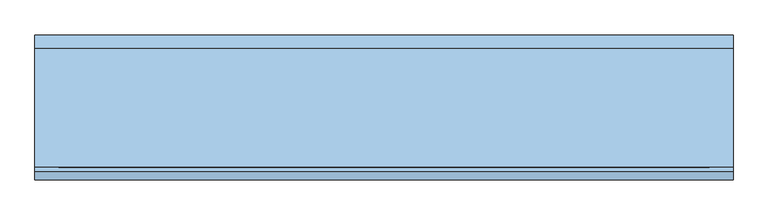
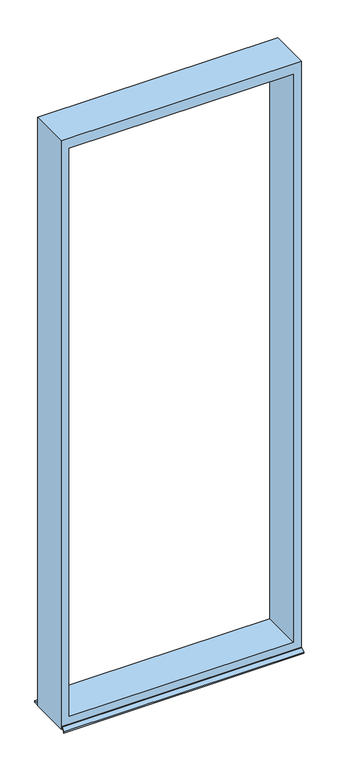
"""IFC4 building model written with IfcOpenShell, lengths in millimetres: window geometry, Fenster - Festverglasung : Feste Verglasung 4.58 x 1.77 3 2 2 2."""

import ifcopenshell
import ifcopenshell.guid

model = None  # the IFC model being written
_history = None  # IfcOwnerHistory: only IFC2X3 demands one
_inside = {}  # id of a spatial element -> (the spatial element, [elements in it])
_under = {}  # id of a project, library or spatial element -> (it, [spatial elements below it])
_declared = {}  # id of a project -> (the project, [libraries it declares])
_typed = {}  # id of a type object -> (the type object, [elements of that type])
_made_of = {}  # id of a material, layer set ... -> (it, [elements and type objects made of it])


def new_model(schema):
    """Start an empty IFC model of exactly this schema.

    Asked for "IFC4X3", IfcOpenShell would pick the latest addendum, in which some entities
    have other attributes; the version numbers below select the first issue.
    IFC2X3 requires an IfcOwnerHistory on every rooted entity: one is made here for all.
    """
    global model, _history
    if schema == "IFC4X3":
        model = ifcopenshell.file(schema_version=(4, 3, 0, 0))
    else:
        model = ifcopenshell.file(schema=schema)
    _inside.clear()
    _under.clear()
    _declared.clear()
    _typed.clear()
    _made_of.clear()
    _history = None
    if model.schema == "IFC2X3":
        org = make("IfcOrganization", Name="unknown")
        user = make(
            "IfcPersonAndOrganization",
            ThePerson=make("IfcPerson", FamilyName="unknown"),
            TheOrganization=org,
        )
        app = make(
            "IfcApplication",
            ApplicationDeveloper=org,
            Version="unknown",
            ApplicationFullName="unknown",
            ApplicationIdentifier="unknown",
        )
        _history = make(
            "IfcOwnerHistory",
            OwningUser=user,
            OwningApplication=app,
            ChangeAction="ADDED",
            CreationDate=0,
        )
    return model


def make(cls, **values):
    """One entity of the class cls with the attributes given. An attribute that is None is left unset."""
    return model.create_entity(
        cls, **{name: value for name, value in values.items() if value is not None}
    )


def rooted(cls, **values):
    """An entity with a GlobalId (a new one), such as an element, a storey or a relation."""
    return make(cls, GlobalId=ifcopenshell.guid.new(), OwnerHistory=_history, **values)


def si_unit(unit_type, name, prefix=None):
    """IfcSIUnit, for example si_unit("LENGTHUNIT", "METRE", prefix="MILLI")."""
    return make("IfcSIUnit", UnitType=unit_type, Prefix=prefix, Name=name)


def assignment(units):
    """IfcUnitAssignment: the units of a project."""
    return None if units is None else make("IfcUnitAssignment", Units=units)


def point(xyz):
    """IfcCartesianPoint."""
    return None if xyz is None else make("IfcCartesianPoint", Coordinates=xyz)


def direction(xyz):
    """IfcDirection."""
    return None if xyz is None else make("IfcDirection", DirectionRatios=xyz)


def frame(location, z_axis=None, x_axis=None):
    """IfcAxis2Placement3D, a coordinate frame: its origin and axes. An axis left out is left unset."""
    return make(
        "IfcAxis2Placement3D",
        Location=point(location),
        Axis=direction(z_axis),
        RefDirection=direction(x_axis),
    )


def origin():
    """The frame at (0, 0, 0) with its axes left unset."""
    return frame((0.0, 0.0, 0.0))


def place(relative_to, where):
    """IfcLocalPlacement: puts the frame where relative to a parent placement (None: the world)."""
    return make(
        "IfcLocalPlacement", PlacementRelTo=relative_to, RelativePlacement=where
    )


def context(
    kind, dimensions, precision=None, world=None, true_north=None, identifier=None
):
    """IfcGeometricRepresentationContext, for example the 3D "Model" context."""
    return make(
        "IfcGeometricRepresentationContext",
        ContextIdentifier=identifier,
        ContextType=kind,
        CoordinateSpaceDimension=dimensions,
        Precision=precision,
        WorldCoordinateSystem=world,
        TrueNorth=true_north,
    )


def project(units=None, contexts=None):
    """IfcProject with its units and contexts."""
    return rooted(
        "IfcProject",
        Name="project",
        RepresentationContexts=contexts,
        UnitsInContext=assignment(units),
    )


def spatial(cls, under=None, at=None, **own):
    """A site, building, storey or space (cls), placed at a placement, below another one or the project."""
    s = rooted(cls, ObjectPlacement=at, **own)
    if under is not None:
        _under.setdefault(under.id(), (under, []))[1].append(s)
    return s


def polyline(points):
    """IfcPolyline through the points."""
    return make("IfcPolyline", Points=[point(p) for p in points])


def outline(outer, holes=None, kind="AREA"):
    """IfcArbitraryClosedProfileDef: a profile drawn as a closed curve; with holes, ...WithVoids."""
    if holes is None:
        return make("IfcArbitraryClosedProfileDef", ProfileType=kind, OuterCurve=outer)
    return make(
        "IfcArbitraryProfileDefWithVoids",
        ProfileType=kind,
        OuterCurve=outer,
        InnerCurves=holes,
    )


def extrude(swept, where, along, depth):
    """IfcExtrudedAreaSolid: the profile swept, set in the frame where, extruded along a direction by depth."""
    return make(
        "IfcExtrudedAreaSolid",
        SweptArea=swept,
        Position=where,
        ExtrudedDirection=direction(along),
        Depth=depth,
    )


def shape(context_of_items, identifier, shape_type, items):
    """IfcShapeRepresentation: the items that make up one representation, for example the "Body"."""
    return make(
        "IfcShapeRepresentation",
        ContextOfItems=context_of_items,
        RepresentationIdentifier=identifier,
        RepresentationType=shape_type,
        Items=items,
    )


def source(mapping_origin, context_of_items, identifier, shape_type, items):
    """IfcRepresentationMap: a shape defined once, which mapped items show again and again."""
    return make(
        "IfcRepresentationMap",
        MappingOrigin=mapping_origin,
        MappedRepresentation=shape(context_of_items, identifier, shape_type, items),
    )


def transform(
    local_origin,
    x_axis=None,
    y_axis=None,
    z_axis=None,
    scale=None,
    scale2=None,
    scale3=None,
    uniform=True,
):
    """IfcCartesianTransformationOperator3D, or its non-uniform kind. x_axis, y_axis, z_axis: its Axis1, 2, 3."""
    if uniform:
        return make(
            "IfcCartesianTransformationOperator3D",
            Axis1=direction(x_axis),
            Axis2=direction(y_axis),
            LocalOrigin=point(local_origin),
            Scale=scale,
            Axis3=direction(z_axis),
        )
    return make(
        "IfcCartesianTransformationOperator3DnonUniform",
        Axis1=direction(x_axis),
        Axis2=direction(y_axis),
        LocalOrigin=point(local_origin),
        Scale=scale,
        Axis3=direction(z_axis),
        Scale2=scale2,
        Scale3=scale3,
    )


def mapped(mapping_source, mapping_target):
    """IfcMappedItem: shows the shape of a source again, moved by a transform."""
    return make(
        "IfcMappedItem", MappingSource=mapping_source, MappingTarget=mapping_target
    )


def made_of(thing, what):
    """Note that an element or type object is made of a material, layer set ...; save() writes the relation."""
    if what is not None:
        _made_of.setdefault(what.id(), (what, []))[1].append(thing)
    return thing


def element(
    cls,
    number,
    at=None,
    inside=None,
    cuts=None,
    type_object=None,
    material=None,
    context=None,
    identifier="Body",
    shape_type=None,
    held_by="IfcProductDefinitionShape",
    body=None,
    shapes=None,
    **own,
):
    """One element of the class cls, such as IfcWall. Its Tag is "e" and its number.

    at: its placement. inside: the storey or other place that contains it. cuts: it is an
    opening in that element (IfcRelVoidsElement). A single representation is given by context,
    identifier, shape_type and body (its items); several are given by shapes. held_by: the class
    of the entity that holds the representations. save() writes the other relations.
    """
    e = rooted(cls, Tag="e%d" % number, ObjectPlacement=at, **own)
    if body is not None:
        shapes = [shape(context, identifier, shape_type, body)]
    if shapes is not None:
        e.Representation = make(held_by, Representations=shapes)
    if inside is not None:
        _inside.setdefault(inside.id(), (inside, []))[1].append(e)
    if cuts is not None:
        rooted(
            "IfcRelVoidsElement", RelatingBuildingElement=cuts, RelatedOpeningElement=e
        )
    if type_object is not None:
        _typed.setdefault(type_object.id(), (type_object, []))[1].append(e)
    return made_of(e, material)


def aggregate(whole, parts):
    """IfcRelAggregates: a whole, such as a stair, and the parts it consists of."""
    return rooted("IfcRelAggregates", RelatingObject=whole, RelatedObjects=parts)


def save(model, path):
    """Write the relations noted so far, then the file.

    IfcRelAggregates (storeys below a building ...), IfcRelContainedInSpatialStructure (elements
    in a storey), IfcRelDefinesByType, IfcRelAssociatesMaterial and IfcRelDeclares: one each for
    every whole, place, type object, material and project.
    """
    for whole, parts in _under.values():
        aggregate(whole, parts)
    for where, things in _inside.values():
        rooted(
            "IfcRelContainedInSpatialStructure",
            RelatedElements=things,
            RelatingStructure=where,
        )
    for kind, things in _typed.values():
        rooted("IfcRelDefinesByType", RelatedObjects=things, RelatingType=kind)
    for what, things in _made_of.values():
        rooted("IfcRelAssociatesMaterial", RelatedObjects=things, RelatingMaterial=what)
    for by, libraries in _declared.values():
        rooted("IfcRelDeclares", RelatingContext=by, RelatedDefinitions=libraries)
    model.write(path)


def window_84ed85f0(model_context):
    return source(origin(), model_context, "Body", "SweptSolid", [
        extrude(outline(polyline([(5580.0, 885.0), (5580.0, -885.0), (1000.0, -885.0), (1000.0, 885.0), (5580.0, 885.0)]), holes=[polyline([(5500.0, 825.0), (1080.0, 825.0), (1080.0, -825.0), (5500.0, -825.0), (5500.0, 825.0)])]), frame((0.0, -151.5214598, 0.0), z_axis=(0.0, 1.0, 0.0), x_axis=(0.0, 0.0, 1.0)), (0.0, 0.0, 1.0), 300.0),
        extrude(outline(polyline([(-885.0, 184.0), (885.0, 184.0), (885.0, 148.4785402), (-885.0, 148.4785402), (-885.0, 184.0)])), frame((0.0, 0.0, 1005.0), z_axis=(0.0, 0.0, 1.0), x_axis=(1.0, 0.0, 0.0)), (0.0, 0.0, 1.0), 15.0),
        extrude(outline(polyline([(-161.5436142, 1020.0), (-151.5214598, 1020.0), (-151.5214598, 1018.0), (-161.3455321, 1018.0), (-182.0, 998.3604634), (-182.0, 990.0), (-184.0, 990.0), (-184.0, 1000.0), (-161.5436142, 1020.0)])), frame((-885.0, 0.0, 0.0), z_axis=(1.0, 0.0, 0.0), x_axis=(0.0, 1.0, 0.0)), (0.0, 0.0, 1.0), 1770.0),
    ])


if __name__ == "__main__":
    model = new_model("IFC4")
    model_context = context("Model", 3, world=origin())
    ifc_project = project(units=[si_unit("LENGTHUNIT", "METRE", prefix="MILLI")], contexts=[model_context])
    site = spatial("IfcSite", under=ifc_project)
    building = spatial("IfcBuilding", under=site)
    placement = place(None, origin())
    window_shape = window_84ed85f0(model_context)
    element("IfcWindow", 1, ObjectType="Fenster - Festverglasung : Feste Verglasung 4.58 x 1.77 3 2 2 2", at=placement, inside=building, context=model_context, shape_type="MappedRepresentation", body=[
        mapped(window_shape, transform((0.0, 0.0, 0.0), x_axis=(1.0, 0.0, 0.0), y_axis=(0.0, 1.0, 0.0), z_axis=(0.0, 0.0, 1.0))),
    ])
    save(model, "model.ifc")

# Revit data of these elements
# Type "Fenster - Festverglasung : Feste Verglasung 4.58 x 1.77 3 2 2 2"
#   Type Mark = "68"
#   Operation = "SinglePanel"
#   Keynote = "16.05.01"
#   Visual Light Transmittance = 0.9
#   Solar Heat Gain Coefficient = 0.78
#   Rough Width = 1.770 m
#   Rough Height = 4.580 m
#   Heat Transfer Coefficient (U) = 3.6886 W/(m²·K)
#   Rahmentiefe = 0.300 m
#   Rahmenhöhe unten = 0.080 m
#   Höhe oberer  Rahmen = 0.080 m
#   Rahmenbreite = 0.060 m
#   Height = 4.580 m
#   Einbautiefe (von außen) [instance default] = 0.080 m
#   Width = 1.770 m
#   Wall Closure = 3
#   Bild [instance default] = none
#   Glas [instance default] = none
#   Innere Fensterbank [instance default] = none
#   Äußere Fensterbank [instance default] = none
#   Construction Type Id = ""
#   Analytic Construction = (empty or 0)
# Element 1 (IfcWindow, "Fenster - Festverglasung : Feste Verglasung 4.58 x 1.77 3 2 2 2")
#   Einbautiefe (von außen) = 0.002479 m
#   Materials on its faces: "Kunststoff - Weiß", "Holz - Birke"
# Materials
#   "Kunststoff - Weiß": class "Kunststoff", colour RGB 249 249 249, transparency 0, Cost = 0
#   "Holz - Birke": class "Holz", colour RGB 213 164 103, transparency 0, Cost = 0
